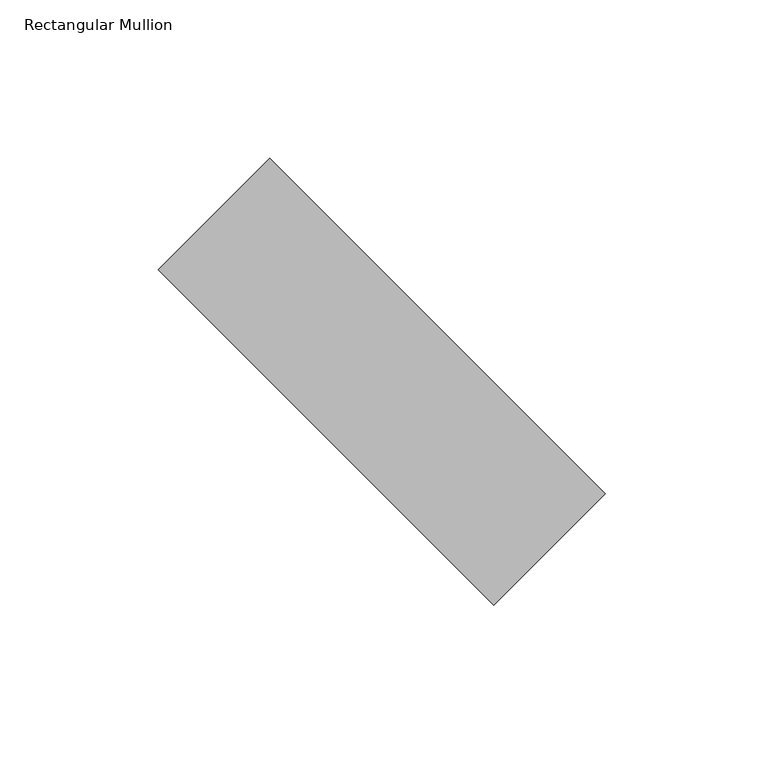
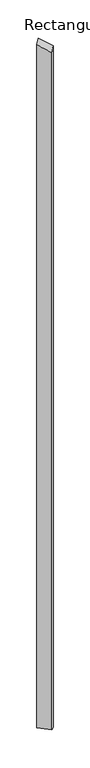
"""IFC4 building model written with IfcOpenShell, lengths in millimetres: member geometry, Rectangular Mullion : tilted mullions."""

from ifc_helpers import new_model, si_unit, origin, place, context, project, spatial, faceted_brep, source, transform, mapped, element, save


def rectangular_mullion_5539c6e3(model_context):
    return source(origin(), model_context, "Body", "Brep", [
        faceted_brep([(-35.3553391, 70.7106781, -7999.4755006), (70.7106781, -35.3553391, -7999.4755006), (35.3553391, -70.7106781, -7999.4755006), (-70.7106781, 35.3553391, -7999.4755006), (-70.7106781, 35.3553391, 10.1551702), (-35.3553391, 70.7106781, 55.165332), (35.3553391, -70.7106781, -55.165332), (70.7106781, -35.3553391, -10.1551702)], [[[0, 1, 2, 3]], [[4, 5, 0, 3]], [[6, 4, 3, 2]], [[7, 6, 2, 1]], [[5, 7, 1, 0]], [[5, 4, 6, 7]]]),
    ])


if __name__ == "__main__":
    model = new_model("IFC4")
    model_context = context("Model", 3, world=origin())
    ifc_project = project(units=[si_unit("LENGTHUNIT", "METRE", prefix="MILLI")], contexts=[model_context])
    site = spatial("IfcSite", under=ifc_project)
    building = spatial("IfcBuilding", under=site)
    placement = place(None, origin())
    rectangular_mullion_shape = rectangular_mullion_5539c6e3(model_context)
    element("IfcMember", 1, ObjectType="Rectangular Mullion : tilted mullions", at=placement, inside=building, context=model_context, shape_type="MappedRepresentation", body=[
        mapped(rectangular_mullion_shape, transform((0.0, 0.0, 0.0), x_axis=(1.0, 0.0, 0.0), y_axis=(0.0, 1.0, 0.0), z_axis=(0.0, 0.0, 1.0))),
    ])
    save(model, "model.ifc")

# Revit data of these elements
# Type "Rectangular Mullion : tilted mullions"
#   built-in parameter 1007304 = 0.492126 (stored number, unit not read)
#   built-in parameter 1007301 = 0.082021 (stored number, unit not read)
#   built-in parameter 1007300 = 0.082021 (stored number, unit not read)
# Element 1 (IfcMember, "Rectangular Mullion : tilted mullions")
#   Materials on its faces: "Aluminum"
# Materials
#   "Aluminum": class "Metal", colour RGB 244 244 244, transparency 0, Description = "Aluminum 6061", Cost = 0
